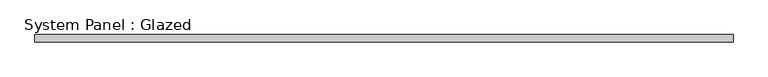
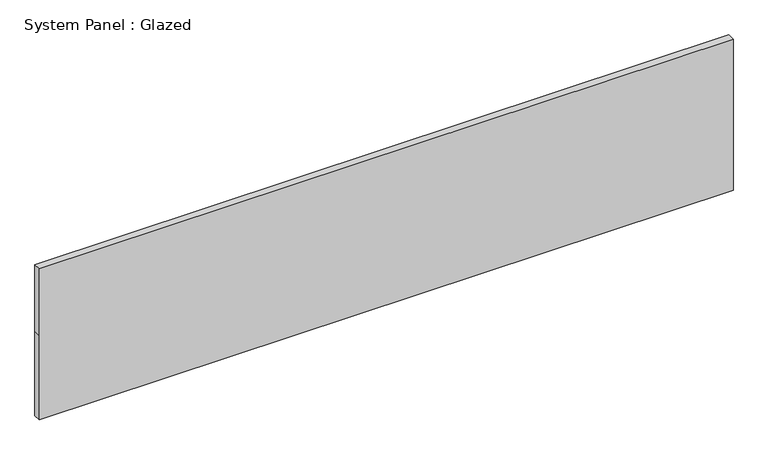
"""IFC4 building model written with IfcOpenShell, lengths in millimetres: plate geometry, System Panel : Glazed."""

import ifcopenshell
import ifcopenshell.guid

model = None  # the IFC model being written
_history = None  # IfcOwnerHistory: only IFC2X3 demands one
_inside = {}  # id of a spatial element -> (the spatial element, [elements in it])
_under = {}  # id of a project, library or spatial element -> (it, [spatial elements below it])
_declared = {}  # id of a project -> (the project, [libraries it declares])
_typed = {}  # id of a type object -> (the type object, [elements of that type])
_made_of = {}  # id of a material, layer set ... -> (it, [elements and type objects made of it])


def new_model(schema):
    """Start an empty IFC model of exactly this schema.

    Asked for "IFC4X3", IfcOpenShell would pick the latest addendum, in which some entities
    have other attributes; the version numbers below select the first issue.
    IFC2X3 requires an IfcOwnerHistory on every rooted entity: one is made here for all.
    """
    global model, _history
    if schema == "IFC4X3":
        model = ifcopenshell.file(schema_version=(4, 3, 0, 0))
    else:
        model = ifcopenshell.file(schema=schema)
    _inside.clear()
    _under.clear()
    _declared.clear()
    _typed.clear()
    _made_of.clear()
    _history = None
    if model.schema == "IFC2X3":
        org = make("IfcOrganization", Name="unknown")
        user = make(
            "IfcPersonAndOrganization",
            ThePerson=make("IfcPerson", FamilyName="unknown"),
            TheOrganization=org,
        )
        app = make(
            "IfcApplication",
            ApplicationDeveloper=org,
            Version="unknown",
            ApplicationFullName="unknown",
            ApplicationIdentifier="unknown",
        )
        _history = make(
            "IfcOwnerHistory",
            OwningUser=user,
            OwningApplication=app,
            ChangeAction="ADDED",
            CreationDate=0,
        )
    return model


def make(cls, **values):
    """One entity of the class cls with the attributes given. An attribute that is None is left unset."""
    return model.create_entity(
        cls, **{name: value for name, value in values.items() if value is not None}
    )


def rooted(cls, **values):
    """An entity with a GlobalId (a new one), such as an element, a storey or a relation."""
    return make(cls, GlobalId=ifcopenshell.guid.new(), OwnerHistory=_history, **values)


def si_unit(unit_type, name, prefix=None):
    """IfcSIUnit, for example si_unit("LENGTHUNIT", "METRE", prefix="MILLI")."""
    return make("IfcSIUnit", UnitType=unit_type, Prefix=prefix, Name=name)


def assignment(units):
    """IfcUnitAssignment: the units of a project."""
    return None if units is None else make("IfcUnitAssignment", Units=units)


def point(xyz):
    """IfcCartesianPoint."""
    return None if xyz is None else make("IfcCartesianPoint", Coordinates=xyz)


def direction(xyz):
    """IfcDirection."""
    return None if xyz is None else make("IfcDirection", DirectionRatios=xyz)


def frame(location, z_axis=None, x_axis=None):
    """IfcAxis2Placement3D, a coordinate frame: its origin and axes. An axis left out is left unset."""
    return make(
        "IfcAxis2Placement3D",
        Location=point(location),
        Axis=direction(z_axis),
        RefDirection=direction(x_axis),
    )


def origin():
    """The frame at (0, 0, 0) with its axes left unset."""
    return frame((0.0, 0.0, 0.0))


def place(relative_to, where):
    """IfcLocalPlacement: puts the frame where relative to a parent placement (None: the world)."""
    return make(
        "IfcLocalPlacement", PlacementRelTo=relative_to, RelativePlacement=where
    )


def context(
    kind, dimensions, precision=None, world=None, true_north=None, identifier=None
):
    """IfcGeometricRepresentationContext, for example the 3D "Model" context."""
    return make(
        "IfcGeometricRepresentationContext",
        ContextIdentifier=identifier,
        ContextType=kind,
        CoordinateSpaceDimension=dimensions,
        Precision=precision,
        WorldCoordinateSystem=world,
        TrueNorth=true_north,
    )


def project(units=None, contexts=None):
    """IfcProject with its units and contexts."""
    return rooted(
        "IfcProject",
        Name="project",
        RepresentationContexts=contexts,
        UnitsInContext=assignment(units),
    )


def spatial(cls, under=None, at=None, **own):
    """A site, building, storey or space (cls), placed at a placement, below another one or the project."""
    s = rooted(cls, ObjectPlacement=at, **own)
    if under is not None:
        _under.setdefault(under.id(), (under, []))[1].append(s)
    return s


def polyline(points):
    """IfcPolyline through the points."""
    return make("IfcPolyline", Points=[point(p) for p in points])


def outline(outer, holes=None, kind="AREA"):
    """IfcArbitraryClosedProfileDef: a profile drawn as a closed curve; with holes, ...WithVoids."""
    if holes is None:
        return make("IfcArbitraryClosedProfileDef", ProfileType=kind, OuterCurve=outer)
    return make(
        "IfcArbitraryProfileDefWithVoids",
        ProfileType=kind,
        OuterCurve=outer,
        InnerCurves=holes,
    )


def extrude(swept, where, along, depth):
    """IfcExtrudedAreaSolid: the profile swept, set in the frame where, extruded along a direction by depth."""
    return make(
        "IfcExtrudedAreaSolid",
        SweptArea=swept,
        Position=where,
        ExtrudedDirection=direction(along),
        Depth=depth,
    )


def shape(context_of_items, identifier, shape_type, items):
    """IfcShapeRepresentation: the items that make up one representation, for example the "Body"."""
    return make(
        "IfcShapeRepresentation",
        ContextOfItems=context_of_items,
        RepresentationIdentifier=identifier,
        RepresentationType=shape_type,
        Items=items,
    )


def source(mapping_origin, context_of_items, identifier, shape_type, items):
    """IfcRepresentationMap: a shape defined once, which mapped items show again and again."""
    return make(
        "IfcRepresentationMap",
        MappingOrigin=mapping_origin,
        MappedRepresentation=shape(context_of_items, identifier, shape_type, items),
    )


def transform(
    local_origin,
    x_axis=None,
    y_axis=None,
    z_axis=None,
    scale=None,
    scale2=None,
    scale3=None,
    uniform=True,
):
    """IfcCartesianTransformationOperator3D, or its non-uniform kind. x_axis, y_axis, z_axis: its Axis1, 2, 3."""
    if uniform:
        return make(
            "IfcCartesianTransformationOperator3D",
            Axis1=direction(x_axis),
            Axis2=direction(y_axis),
            LocalOrigin=point(local_origin),
            Scale=scale,
            Axis3=direction(z_axis),
        )
    return make(
        "IfcCartesianTransformationOperator3DnonUniform",
        Axis1=direction(x_axis),
        Axis2=direction(y_axis),
        LocalOrigin=point(local_origin),
        Scale=scale,
        Axis3=direction(z_axis),
        Scale2=scale2,
        Scale3=scale3,
    )


def mapped(mapping_source, mapping_target):
    """IfcMappedItem: shows the shape of a source again, moved by a transform."""
    return make(
        "IfcMappedItem", MappingSource=mapping_source, MappingTarget=mapping_target
    )


def made_of(thing, what):
    """Note that an element or type object is made of a material, layer set ...; save() writes the relation."""
    if what is not None:
        _made_of.setdefault(what.id(), (what, []))[1].append(thing)
    return thing


def element(
    cls,
    number,
    at=None,
    inside=None,
    cuts=None,
    type_object=None,
    material=None,
    context=None,
    identifier="Body",
    shape_type=None,
    held_by="IfcProductDefinitionShape",
    body=None,
    shapes=None,
    **own,
):
    """One element of the class cls, such as IfcWall. Its Tag is "e" and its number.

    at: its placement. inside: the storey or other place that contains it. cuts: it is an
    opening in that element (IfcRelVoidsElement). A single representation is given by context,
    identifier, shape_type and body (its items); several are given by shapes. held_by: the class
    of the entity that holds the representations. save() writes the other relations.
    """
    e = rooted(cls, Tag="e%d" % number, ObjectPlacement=at, **own)
    if body is not None:
        shapes = [shape(context, identifier, shape_type, body)]
    if shapes is not None:
        e.Representation = make(held_by, Representations=shapes)
    if inside is not None:
        _inside.setdefault(inside.id(), (inside, []))[1].append(e)
    if cuts is not None:
        rooted(
            "IfcRelVoidsElement", RelatingBuildingElement=cuts, RelatedOpeningElement=e
        )
    if type_object is not None:
        _typed.setdefault(type_object.id(), (type_object, []))[1].append(e)
    return made_of(e, material)


def aggregate(whole, parts):
    """IfcRelAggregates: a whole, such as a stair, and the parts it consists of."""
    return rooted("IfcRelAggregates", RelatingObject=whole, RelatedObjects=parts)


def save(model, path):
    """Write the relations noted so far, then the file.

    IfcRelAggregates (storeys below a building ...), IfcRelContainedInSpatialStructure (elements
    in a storey), IfcRelDefinesByType, IfcRelAssociatesMaterial and IfcRelDeclares: one each for
    every whole, place, type object, material and project.
    """
    for whole, parts in _under.values():
        aggregate(whole, parts)
    for where, things in _inside.values():
        rooted(
            "IfcRelContainedInSpatialStructure",
            RelatedElements=things,
            RelatingStructure=where,
        )
    for kind, things in _typed.values():
        rooted("IfcRelDefinesByType", RelatedObjects=things, RelatingType=kind)
    for what, things in _made_of.values():
        rooted("IfcRelAssociatesMaterial", RelatedObjects=things, RelatingMaterial=what)
    for by, libraries in _declared.values():
        rooted("IfcRelDeclares", RelatingContext=by, RelatedDefinitions=libraries)
    model.write(path)


def system_panel_glazed_75890ef7(model_context):
    return source(origin(), model_context, "Body", "SweptSolid", [
        extrude(outline(polyline([(0.0, -1187.45), (0.0, 1187.45), (304.8, 1187.45), (546.1, 1187.45), (546.1, -1187.45), (304.8, -1187.45), (0.0, -1187.45)])), frame((0.0, -44.45, 0.0), z_axis=(0.0, 1.0, 0.0), x_axis=(0.0, 0.0, 1.0)), (0.0, 0.0, 1.0), 25.4),
    ])


if __name__ == "__main__":
    model = new_model("IFC4")
    model_context = context("Model", 3, world=origin())
    ifc_project = project(units=[si_unit("LENGTHUNIT", "METRE", prefix="MILLI")], contexts=[model_context])
    site = spatial("IfcSite", under=ifc_project)
    building = spatial("IfcBuilding", under=site)
    placement = place(None, origin())
    system_panel_glazed_shape = system_panel_glazed_75890ef7(model_context)
    element("IfcPlate", 1, ObjectType="System Panel : Glazed", at=placement, inside=building, context=model_context, shape_type="MappedRepresentation", body=[
        mapped(system_panel_glazed_shape, transform((0.0, 0.0, 0.0), x_axis=(1.0, 0.0, 0.0), y_axis=(0.0, 1.0, 0.0), z_axis=(0.0, 0.0, 1.0))),
    ])
    save(model, "model.ifc")

# Revit data of these elements
# Element 1 (IfcPlate, "System Panel : Glazed")
#   Materials on its faces: "Glass"
# Materials
#   "Glass": class "Glass", colour RGB 0 128 192, transparency 0.75
